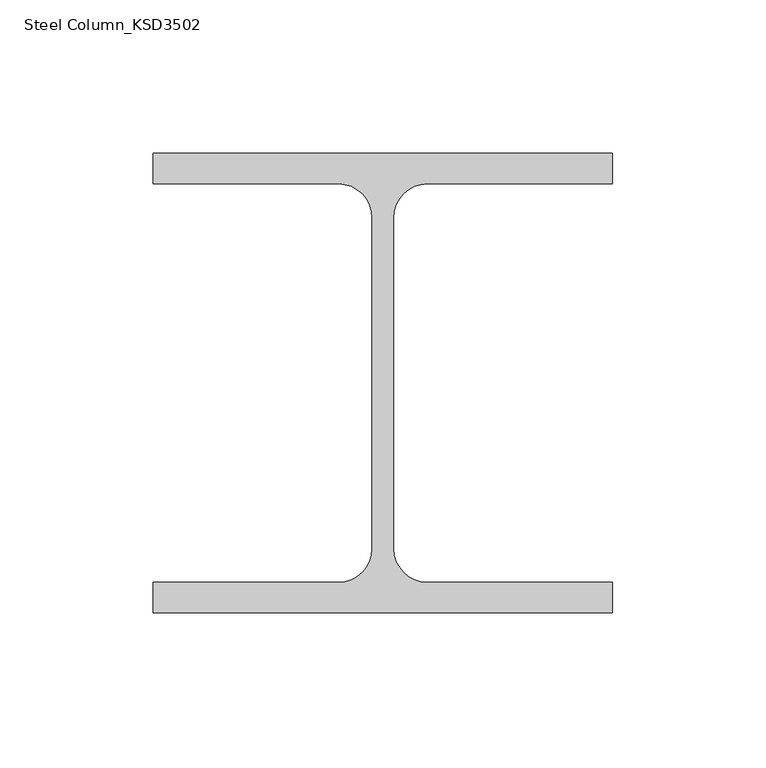
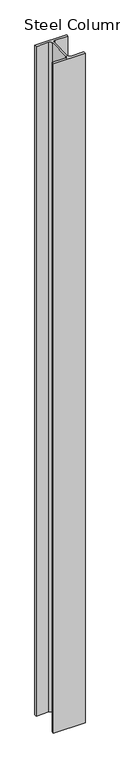
"""IFC4 building model written with IfcOpenShell, lengths in millimetres: column geometry, Steel Column_KSD3502 : H_SC_ASC_H-150×150x7x10."""

from ifc_helpers import new_model, si_unit, point, frame, frame_2d, origin, place, context, project, spatial, polyline, circle_curve, trimmed, segment, composite_curve, outline, extrude, source, transform, mapped, element, save


def steel_column_ksd3502_ee857ed7(model_context):
    return source(origin(), model_context, "Body", "SweptSolid", [
        extrude(outline(composite_curve([segment(polyline([(75.0, 75.0), (75.0, 65.0), (14.5, 65.0)]), True, "CONTINUOUS"), segment(trimmed(circle_curve(frame_2d((14.5, 54.0)), 11.0), [point((14.5, 65.0))], [point((3.5, 54.0))], True, "CARTESIAN"), True, "CONTINUOUS"), segment(polyline([(3.5, 54.0), (3.5, -54.0)]), True, "CONTINUOUS"), segment(trimmed(circle_curve(frame_2d((14.5, -54.0)), 11.0), [point((3.5, -54.0))], [point((14.5, -65.0))], True, "CARTESIAN"), True, "CONTINUOUS"), segment(polyline([(14.5, -65.0), (75.0, -65.0), (75.0, -75.0), (-75.0, -75.0), (-75.0, -65.0), (-14.5, -65.0)]), True, "CONTINUOUS"), segment(trimmed(circle_curve(frame_2d((-14.5, -54.0)), 11.0), [point((-14.5, -65.0))], [point((-3.5, -54.0))], True, "CARTESIAN"), True, "CONTINUOUS"), segment(polyline([(-3.5, -54.0), (-3.5, 54.0)]), True, "CONTINUOUS"), segment(trimmed(circle_curve(frame_2d((-14.5, 54.0)), 11.0), [point((-3.5, 54.0))], [point((-14.5, 65.0))], True, "CARTESIAN"), True, "CONTINUOUS"), segment(polyline([(-14.5, 65.0), (-75.0, 65.0), (-75.0, 75.0), (75.0, 75.0)]), True, "CONTINUOUS")], self_intersect=False)), frame((0.0, 0.0, 4617.9720055), z_axis=(0.0, 0.0, 1.0), x_axis=(1.0, 0.0, 0.0)), (0.0, 0.0, 1.0), 3342.0),
    ])


if __name__ == "__main__":
    model = new_model("IFC4")
    model_context = context("Model", 3, world=origin())
    ifc_project = project(units=[si_unit("LENGTHUNIT", "METRE", prefix="MILLI")], contexts=[model_context])
    site = spatial("IfcSite", under=ifc_project)
    building = spatial("IfcBuilding", under=site)
    placement = place(None, origin())
    steel_column_ksd3502_shape = steel_column_ksd3502_ee857ed7(model_context)
    element("IfcColumn", 1, ObjectType="Steel Column_KSD3502 : H_SC_ASC_H-150×150x7x10", at=placement, inside=building, context=model_context, shape_type="MappedRepresentation", body=[
        mapped(steel_column_ksd3502_shape, transform((0.0, 0.0, 0.0), x_axis=(1.0, 0.0, 0.0), y_axis=(0.0, 1.0, 0.0), z_axis=(0.0, 0.0, 1.0))),
    ])
    save(model, "model.ifc")

# Revit data of these elements
# Type "Steel Column_KSD3502 : H_SC_ASC_H-150×150x7x10"
#   Width = 15.0 cm
#   Web Thickness = 0.7 cm
#   Web Fillet = 1.1 cm
#   Warping Constant = 27562.5 cm⁶
#   Torsional Moment of Inertia = 11.6007 cm⁴
#   Section Area = 40.14 cm²
#   Plastic Modulus weak axis = 115.0 cm³
#   Plastic Modulus strong axis = 246.0 cm³
#   Perimeter = 1.27 m²/m
#   Nominal Weight = 31.50 kgf/m
#   Moment of Inertia weak axis = 563.00 cm⁴
#   Moment of Inertia strong axis = 1640.00 cm⁴
#   Height = 15.0 cm
#   Flange Thickness = 1.0 cm
#   Elastic Modulus weak axis = 75.1 cm³
#   Elastic Modulus strong axis = 219.0 cm³
#   Centroid Vertical = 7.5 cm
#   Centroid Horizontal = 7.5 cm
#   Bolt Spacing = 13.97 cm
#   Structural Material [instance default] = Steel, 45-345
#   Section Name Key = ""
#   Assembly Code = ""
# Element 1 (IfcColumn, "Steel Column_KSD3502 : H_SC_ASC_H-150×150x7x10")
#   Structural Material = none
# Materials
#   "Steel, 45-345": class "Metal", colour RGB 189 187 185, transparency 0, Description = "Steel 345 MPa", Cost = 0
